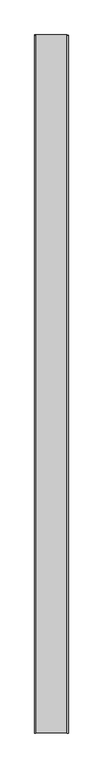
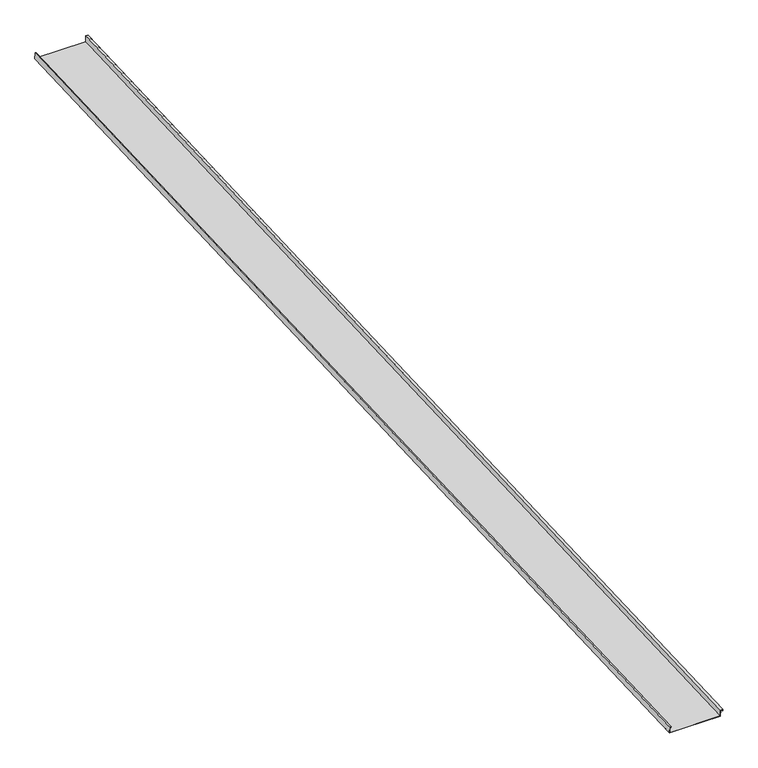
"""IFC4 building model written with IfcOpenShell, lengths in millimetres: proxy geometry, Generic Models 2:Generic Models 2:310765:Generic Models 2:310765 : Generic Models 2:Generic Models 2:310765:200 : Generic Models 2:Generic Models 2:310765:Generic Models 2:310765 : Generic Models 2:Generic Models 2:310765:300385."""

from ifc_helpers import new_model, si_unit, frame, origin, place, context, project, spatial, polyline, outline, extrude, source, transform, mapped, element, save


def generic_models_5061953d(model_context):
    return source(origin(), model_context, "Body", "SweptSolid", [
        extrude(outline(polyline([(50.8, 0.0), (50.8, 14.2875), (41.275, 14.2875), (41.275, 15.875), (52.3874999, 15.875), (52.3874999, -1.5875), (1.5874999, -1.5875), (1.5874999, -404.8125), (47.625, -404.8125), (47.625, -396.875), (39.6875, -396.875), (39.6875, -395.2875), (49.2124999, -395.2875), (49.2124999, -406.4), (0.0, -406.4), (0.0, 0.0), (50.8, 0.0)])), frame((580020.2953039, -581447.5605462, 3847.9454697), z_axis=(0.0, 0.9991330730923567, 0.04163054471206783), x_axis=(0.0, -0.04163054471206783, 0.9991330730923567)), (0.0, 0.0, 1.0), 8776.7038972),
    ])


if __name__ == "__main__":
    model = new_model("IFC4")
    model_context = context("Model", 3, world=origin())
    ifc_project = project(units=[si_unit("LENGTHUNIT", "METRE", prefix="MILLI")], contexts=[model_context])
    site = spatial("IfcSite", under=ifc_project)
    building = spatial("IfcBuilding", under=site)
    placement = place(None, origin())
    generic_models_shape = generic_models_5061953d(model_context)
    element("IfcBuildingElementProxy", 1, Name="Generic Models 2:Generic Models 2:310765:Generic Models 2:310765 : Generic Models 2:Generic Models 2:310765:200 : Generic Models 2:Generic Models 2:310765:Generic Models 2:310765 : Generic Models 2:Generic Models 2:310765:300385", ObjectType="Generic Models 2:Generic Models 2:310765:Generic Models 2:310765 : Generic Models 2:Generic Models 2:310765:200 : Generic Models 2:Generic Models 2:310765:Generic Models 2:310765 : Generic Models 2:Generic Models 2:310765:300385", at=placement, inside=building, context=model_context, shape_type="MappedRepresentation", body=[
        mapped(generic_models_shape, transform((0.0, 0.0, 0.0), x_axis=(1.0, 0.0, 0.0), y_axis=(0.0, 1.0, 0.0), z_axis=(0.0, 0.0, 1.0))),
    ])
    save(model, "model.ifc")

# Revit data of these elements
# Type "Generic Models 2:Generic Models 2:310765:Generic Models 2:310765 : Generic Models 2:Generic Models 2:310765:200 : Generic Models 2:Generic Models 2:310765:Generic Models 2:310765 : Generic Models 2:Generic Models 2:310765:300385"
#   NameOverride = "Generic Models 2:Generic Models 2:310765:Generic Models 2:310765 : Generic Models 2:Generic Models 2:310765:300385"
#   ObjectTypeOverride = "Generic Models 2:310765 : Generic Models 2:Generic Models 2:310765"
#   Reference = "Generic Models 2"
#   Tag = "300385"
# Element 1 (IfcBuildingElementProxy, "Generic Models 2:Generic Models 2:310765:Generic Models 2:310765 : Generic Models 2:Generic Models 2:310765:200 : Generic Models 2:Generic Models 2:310765:Generic Models 2:310765 : Generic Models 2:Generic Models 2:310765:300385")
#   Materials on its faces: "THERMAL BROKEN ALUMINUM STOREFRONT FOR POLYCARBONATE"
# Materials
#   "THERMAL BROKEN ALUMINUM STOREFRONT FOR POLYCARBONATE": class "Unassigned", colour RGB 244 244 244, transparency 0, Keynote = "M07611300.01", Cost = 0
